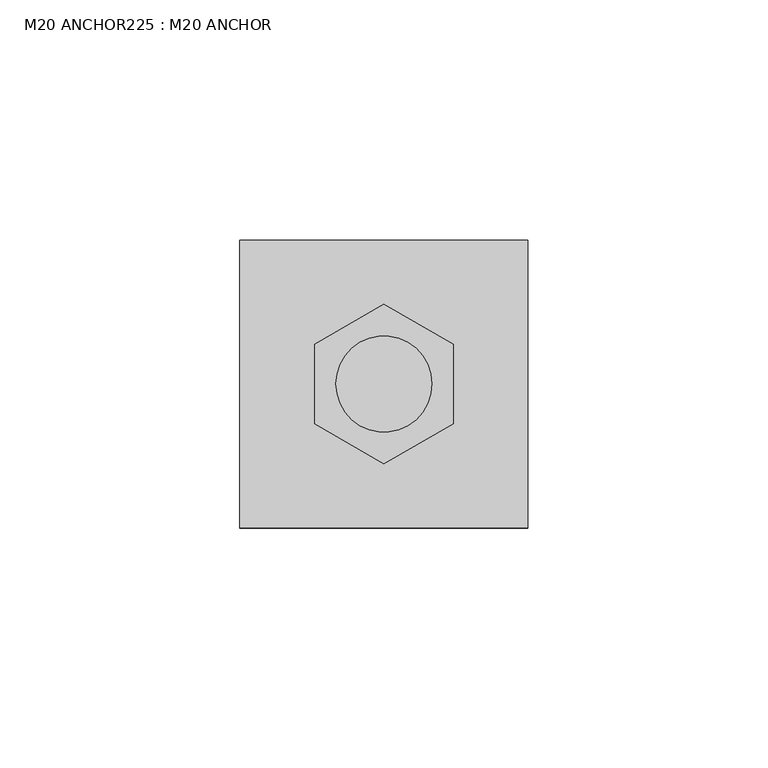
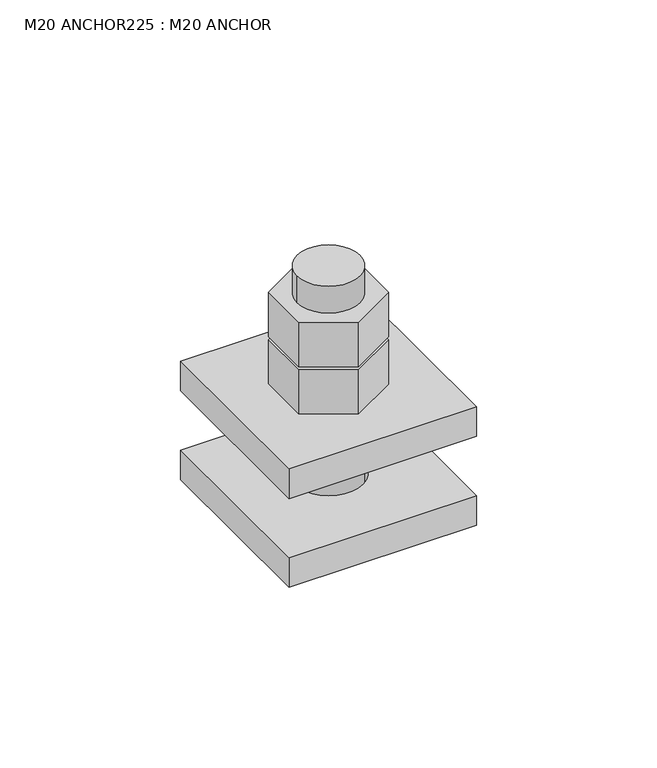
"""IFC4 building model written with IfcOpenShell, lengths in millimetres: fastener geometry, M20 ANCHOR225 : M20 ANCHOR."""

from ifc_helpers import new_model, si_unit, point, frame, frame_2d, origin, place, context, project, spatial, polyline, circle_curve, trimmed, segment, composite_curve, outline, extrude, source, transform, mapped, element, save


def m20_anchor225_m20_anchor_809aad72(model_context):
    return source(origin(), model_context, "Body", "SweptSolid", [
        extrude(outline(polyline([(9008.0855968, 19453.9464399), (9008.0855968, 19470.5835027), (9022.4937158, 19478.9020341), (9036.9018348, 19470.5835027), (9036.9018348, 19453.9464399), (9022.4937158, 19445.6279085), (9008.0855968, 19453.9464399)]), holes=[composite_curve([segment(trimmed(circle_curve(frame_2d((9022.4937158, 19462.2649713)), 10.0), [point((9032.4937158, 19462.2649713))], [point((9012.4937158, 19462.2649713))], True, "CARTESIAN"), True, "CONTINUOUS"), segment(trimmed(circle_curve(frame_2d((9022.4937158, 19462.2649713)), 10.0), [point((9012.4937158, 19462.2649713))], [point((9032.4937158, 19462.2649713))], True, "CARTESIAN"), True, "CONTINUOUS")], self_intersect=False)]), frame((0.0, 0.0, 246.0), z_axis=(0.0, 0.0, 1.0), x_axis=(1.0, 0.0, 0.0)), (0.0, 0.0, 1.0), 15.0),
        extrude(outline(polyline([(9008.0855968, 19453.9464399), (9008.0855968, 19470.5835027), (9022.4937158, 19478.9020341), (9036.9018348, 19470.5835027), (9036.9018348, 19453.9464399), (9022.4937158, 19445.6279085), (9008.0855968, 19453.9464399)]), holes=[composite_curve([segment(trimmed(circle_curve(frame_2d((9022.4937158, 19462.2649713)), 10.0), [point((9032.4937158, 19462.2649713))], [point((9012.4937158, 19462.2649713))], True, "CARTESIAN"), True, "CONTINUOUS"), segment(trimmed(circle_curve(frame_2d((9022.4937158, 19462.2649713)), 10.0), [point((9012.4937158, 19462.2649713))], [point((9032.4937158, 19462.2649713))], True, "CARTESIAN"), True, "CONTINUOUS")], self_intersect=False)]), frame((0.0, 0.0, 230.0), z_axis=(0.0, 0.0, 1.0), x_axis=(1.0, 0.0, 0.0)), (0.0, 0.0, 1.0), 15.0),
        extrude(outline(composite_curve([segment(trimmed(circle_curve(frame_2d((9022.4937158, 19462.2649713)), 10.0), [point((9032.4937158, 19462.2649713))], [point((9012.4937158, 19462.2649713))], False, "CARTESIAN"), True, "CONTINUOUS"), segment(trimmed(circle_curve(frame_2d((9022.4937158, 19462.2649713)), 10.0), [point((9012.4937158, 19462.2649713))], [point((9032.4937158, 19462.2649713))], False, "CARTESIAN"), True, "CONTINUOUS")], self_intersect=False)), frame((0.0, 0.0, 190.0), z_axis=(0.0, 0.0, 1.0), x_axis=(1.0, 0.0, 0.0)), (0.0, 0.0, 1.0), 80.0),
        extrude(outline(polyline([(8992.4937158, 19432.2649713), (8992.4937158, 19492.2649713), (9052.4937158, 19492.2649713), (9052.4937158, 19432.2649713), (8992.4937158, 19432.2649713)]), holes=[composite_curve([segment(trimmed(circle_curve(frame_2d((9022.4937158, 19462.2649713)), 11.0), [point((9033.4937158, 19462.2649713))], [point((9011.4937158, 19462.2649713))], True, "CARTESIAN"), True, "CONTINUOUS"), segment(trimmed(circle_curve(frame_2d((9022.4937158, 19462.2649713)), 11.0), [point((9011.4937158, 19462.2649713))], [point((9033.4937158, 19462.2649713))], True, "CARTESIAN"), True, "CONTINUOUS")], self_intersect=False)]), frame((0.0, 0.0, 190.0), z_axis=(0.0, 0.0, 1.0), x_axis=(1.0, 0.0, 0.0)), (0.0, 0.0, 1.0), 10.0),
        extrude(outline(polyline([(8992.4937158, 19432.2649713), (8992.4937158, 19492.2649713), (9052.4937158, 19492.2649713), (9052.4937158, 19432.2649713), (8992.4937158, 19432.2649713)]), holes=[composite_curve([segment(trimmed(circle_curve(frame_2d((9022.4937158, 19462.2649713)), 11.0), [point((9033.4937158, 19462.2649713))], [point((9011.4937158, 19462.2649713))], True, "CARTESIAN"), True, "CONTINUOUS"), segment(trimmed(circle_curve(frame_2d((9022.4937158, 19462.2649713)), 11.0), [point((9011.4937158, 19462.2649713))], [point((9033.4937158, 19462.2649713))], True, "CARTESIAN"), True, "CONTINUOUS")], self_intersect=False)]), frame((0.0, 0.0, 220.0), z_axis=(0.0, 0.0, 1.0), x_axis=(1.0, 0.0, 0.0)), (0.0, 0.0, 1.0), 10.0),
    ])


if __name__ == "__main__":
    model = new_model("IFC4")
    model_context = context("Model", 3, world=origin())
    ifc_project = project(units=[si_unit("LENGTHUNIT", "METRE", prefix="MILLI")], contexts=[model_context])
    site = spatial("IfcSite", under=ifc_project)
    building = spatial("IfcBuilding", under=site)
    placement = place(None, origin())
    m20_anchor225_m20_anchor_shape = m20_anchor225_m20_anchor_809aad72(model_context)
    element("IfcFastener", 1, ObjectType="M20 ANCHOR225 : M20 ANCHOR", at=placement, inside=building, context=model_context, shape_type="MappedRepresentation", body=[
        mapped(m20_anchor225_m20_anchor_shape, transform((0.0, 0.0, 0.0), x_axis=(1.0, 0.0, 0.0), y_axis=(0.0, 1.0, 0.0), z_axis=(0.0, 0.0, 1.0))),
    ])
    save(model, "model.ifc")
